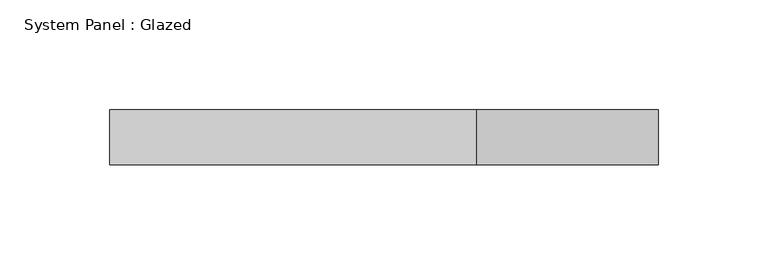
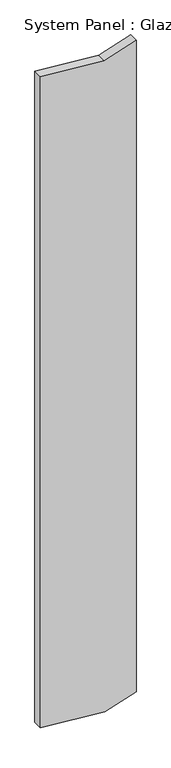
"""IFC4 building model written with IfcOpenShell, lengths in millimetres: plate geometry, System Panel : Glazed."""

import ifcopenshell
import ifcopenshell.guid

model = None  # the IFC model being written
_history = None  # IfcOwnerHistory: only IFC2X3 demands one
_inside = {}  # id of a spatial element -> (the spatial element, [elements in it])
_under = {}  # id of a project, library or spatial element -> (it, [spatial elements below it])
_declared = {}  # id of a project -> (the project, [libraries it declares])
_typed = {}  # id of a type object -> (the type object, [elements of that type])
_made_of = {}  # id of a material, layer set ... -> (it, [elements and type objects made of it])


def new_model(schema):
    """Start an empty IFC model of exactly this schema.

    Asked for "IFC4X3", IfcOpenShell would pick the latest addendum, in which some entities
    have other attributes; the version numbers below select the first issue.
    IFC2X3 requires an IfcOwnerHistory on every rooted entity: one is made here for all.
    """
    global model, _history
    if schema == "IFC4X3":
        model = ifcopenshell.file(schema_version=(4, 3, 0, 0))
    else:
        model = ifcopenshell.file(schema=schema)
    _inside.clear()
    _under.clear()
    _declared.clear()
    _typed.clear()
    _made_of.clear()
    _history = None
    if model.schema == "IFC2X3":
        org = make("IfcOrganization", Name="unknown")
        user = make(
            "IfcPersonAndOrganization",
            ThePerson=make("IfcPerson", FamilyName="unknown"),
            TheOrganization=org,
        )
        app = make(
            "IfcApplication",
            ApplicationDeveloper=org,
            Version="unknown",
            ApplicationFullName="unknown",
            ApplicationIdentifier="unknown",
        )
        _history = make(
            "IfcOwnerHistory",
            OwningUser=user,
            OwningApplication=app,
            ChangeAction="ADDED",
            CreationDate=0,
        )
    return model


def make(cls, **values):
    """One entity of the class cls with the attributes given. An attribute that is None is left unset."""
    return model.create_entity(
        cls, **{name: value for name, value in values.items() if value is not None}
    )


def rooted(cls, **values):
    """An entity with a GlobalId (a new one), such as an element, a storey or a relation."""
    return make(cls, GlobalId=ifcopenshell.guid.new(), OwnerHistory=_history, **values)


def si_unit(unit_type, name, prefix=None):
    """IfcSIUnit, for example si_unit("LENGTHUNIT", "METRE", prefix="MILLI")."""
    return make("IfcSIUnit", UnitType=unit_type, Prefix=prefix, Name=name)


def assignment(units):
    """IfcUnitAssignment: the units of a project."""
    return None if units is None else make("IfcUnitAssignment", Units=units)


def point(xyz):
    """IfcCartesianPoint."""
    return None if xyz is None else make("IfcCartesianPoint", Coordinates=xyz)


def direction(xyz):
    """IfcDirection."""
    return None if xyz is None else make("IfcDirection", DirectionRatios=xyz)


def frame(location, z_axis=None, x_axis=None):
    """IfcAxis2Placement3D, a coordinate frame: its origin and axes. An axis left out is left unset."""
    return make(
        "IfcAxis2Placement3D",
        Location=point(location),
        Axis=direction(z_axis),
        RefDirection=direction(x_axis),
    )


def origin():
    """The frame at (0, 0, 0) with its axes left unset."""
    return frame((0.0, 0.0, 0.0))


def place(relative_to, where):
    """IfcLocalPlacement: puts the frame where relative to a parent placement (None: the world)."""
    return make(
        "IfcLocalPlacement", PlacementRelTo=relative_to, RelativePlacement=where
    )


def context(
    kind, dimensions, precision=None, world=None, true_north=None, identifier=None
):
    """IfcGeometricRepresentationContext, for example the 3D "Model" context."""
    return make(
        "IfcGeometricRepresentationContext",
        ContextIdentifier=identifier,
        ContextType=kind,
        CoordinateSpaceDimension=dimensions,
        Precision=precision,
        WorldCoordinateSystem=world,
        TrueNorth=true_north,
    )


def project(units=None, contexts=None):
    """IfcProject with its units and contexts."""
    return rooted(
        "IfcProject",
        Name="project",
        RepresentationContexts=contexts,
        UnitsInContext=assignment(units),
    )


def spatial(cls, under=None, at=None, **own):
    """A site, building, storey or space (cls), placed at a placement, below another one or the project."""
    s = rooted(cls, ObjectPlacement=at, **own)
    if under is not None:
        _under.setdefault(under.id(), (under, []))[1].append(s)
    return s


def polyline(points):
    """IfcPolyline through the points."""
    return make("IfcPolyline", Points=[point(p) for p in points])


def outline(outer, holes=None, kind="AREA"):
    """IfcArbitraryClosedProfileDef: a profile drawn as a closed curve; with holes, ...WithVoids."""
    if holes is None:
        return make("IfcArbitraryClosedProfileDef", ProfileType=kind, OuterCurve=outer)
    return make(
        "IfcArbitraryProfileDefWithVoids",
        ProfileType=kind,
        OuterCurve=outer,
        InnerCurves=holes,
    )


def extrude(swept, where, along, depth):
    """IfcExtrudedAreaSolid: the profile swept, set in the frame where, extruded along a direction by depth."""
    return make(
        "IfcExtrudedAreaSolid",
        SweptArea=swept,
        Position=where,
        ExtrudedDirection=direction(along),
        Depth=depth,
    )


def shape(context_of_items, identifier, shape_type, items):
    """IfcShapeRepresentation: the items that make up one representation, for example the "Body"."""
    return make(
        "IfcShapeRepresentation",
        ContextOfItems=context_of_items,
        RepresentationIdentifier=identifier,
        RepresentationType=shape_type,
        Items=items,
    )


def source(mapping_origin, context_of_items, identifier, shape_type, items):
    """IfcRepresentationMap: a shape defined once, which mapped items show again and again."""
    return make(
        "IfcRepresentationMap",
        MappingOrigin=mapping_origin,
        MappedRepresentation=shape(context_of_items, identifier, shape_type, items),
    )


def transform(
    local_origin,
    x_axis=None,
    y_axis=None,
    z_axis=None,
    scale=None,
    scale2=None,
    scale3=None,
    uniform=True,
):
    """IfcCartesianTransformationOperator3D, or its non-uniform kind. x_axis, y_axis, z_axis: its Axis1, 2, 3."""
    if uniform:
        return make(
            "IfcCartesianTransformationOperator3D",
            Axis1=direction(x_axis),
            Axis2=direction(y_axis),
            LocalOrigin=point(local_origin),
            Scale=scale,
            Axis3=direction(z_axis),
        )
    return make(
        "IfcCartesianTransformationOperator3DnonUniform",
        Axis1=direction(x_axis),
        Axis2=direction(y_axis),
        LocalOrigin=point(local_origin),
        Scale=scale,
        Axis3=direction(z_axis),
        Scale2=scale2,
        Scale3=scale3,
    )


def mapped(mapping_source, mapping_target):
    """IfcMappedItem: shows the shape of a source again, moved by a transform."""
    return make(
        "IfcMappedItem", MappingSource=mapping_source, MappingTarget=mapping_target
    )


def made_of(thing, what):
    """Note that an element or type object is made of a material, layer set ...; save() writes the relation."""
    if what is not None:
        _made_of.setdefault(what.id(), (what, []))[1].append(thing)
    return thing


def element(
    cls,
    number,
    at=None,
    inside=None,
    cuts=None,
    type_object=None,
    material=None,
    context=None,
    identifier="Body",
    shape_type=None,
    held_by="IfcProductDefinitionShape",
    body=None,
    shapes=None,
    **own,
):
    """One element of the class cls, such as IfcWall. Its Tag is "e" and its number.

    at: its placement. inside: the storey or other place that contains it. cuts: it is an
    opening in that element (IfcRelVoidsElement). A single representation is given by context,
    identifier, shape_type and body (its items); several are given by shapes. held_by: the class
    of the entity that holds the representations. save() writes the other relations.
    """
    e = rooted(cls, Tag="e%d" % number, ObjectPlacement=at, **own)
    if body is not None:
        shapes = [shape(context, identifier, shape_type, body)]
    if shapes is not None:
        e.Representation = make(held_by, Representations=shapes)
    if inside is not None:
        _inside.setdefault(inside.id(), (inside, []))[1].append(e)
    if cuts is not None:
        rooted(
            "IfcRelVoidsElement", RelatingBuildingElement=cuts, RelatedOpeningElement=e
        )
    if type_object is not None:
        _typed.setdefault(type_object.id(), (type_object, []))[1].append(e)
    return made_of(e, material)


def aggregate(whole, parts):
    """IfcRelAggregates: a whole, such as a stair, and the parts it consists of."""
    return rooted("IfcRelAggregates", RelatingObject=whole, RelatedObjects=parts)


def save(model, path):
    """Write the relations noted so far, then the file.

    IfcRelAggregates (storeys below a building ...), IfcRelContainedInSpatialStructure (elements
    in a storey), IfcRelDefinesByType, IfcRelAssociatesMaterial and IfcRelDeclares: one each for
    every whole, place, type object, material and project.
    """
    for whole, parts in _under.values():
        aggregate(whole, parts)
    for where, things in _inside.values():
        rooted(
            "IfcRelContainedInSpatialStructure",
            RelatedElements=things,
            RelatingStructure=where,
        )
    for kind, things in _typed.values():
        rooted("IfcRelDefinesByType", RelatedObjects=things, RelatingType=kind)
    for what, things in _made_of.values():
        rooted("IfcRelAssociatesMaterial", RelatedObjects=things, RelatingMaterial=what)
    for by, libraries in _declared.values():
        rooted("IfcRelDeclares", RelatingContext=by, RelatedDefinitions=libraries)
    model.write(path)


def system_panel_glazed_ad4f34ef(model_context):
    return source(origin(), model_context, "Body", "SweptSolid", [
        extrude(outline(polyline([(14.7138245, -125.0), (0.0, 43.1797838), (27.0254149, 125.0), (1826.3916627, 125.0), (1799.0465952, 42.2120265), (1813.7685539, -125.0), (14.7138245, -125.0)])), frame((0.0, 24.5, 0.0), z_axis=(0.0, 1.0, 0.0), x_axis=(0.0, 0.0, 1.0)), (0.0, 0.0, 1.0), 25.0),
    ])


if __name__ == "__main__":
    model = new_model("IFC4")
    model_context = context("Model", 3, world=origin())
    ifc_project = project(units=[si_unit("LENGTHUNIT", "METRE", prefix="MILLI")], contexts=[model_context])
    site = spatial("IfcSite", under=ifc_project)
    building = spatial("IfcBuilding", under=site)
    placement = place(None, origin())
    system_panel_glazed_shape = system_panel_glazed_ad4f34ef(model_context)
    element("IfcPlate", 1, ObjectType="System Panel : Glazed", at=placement, inside=building, context=model_context, shape_type="MappedRepresentation", body=[
        mapped(system_panel_glazed_shape, transform((0.0, 0.0, 0.0), x_axis=(1.0, 0.0, 0.0), y_axis=(0.0, 1.0, 0.0), z_axis=(0.0, 0.0, 1.0))),
    ])
    save(model, "model.ifc")

# Revit data of these elements
# Element 1 (IfcPlate, "System Panel : Glazed")
#   Materials on its faces: "Glass"
# Materials
#   "Glass": class "Glass", colour RGB 218 227 224, transparency 0.85, Description = "Soda Lime Glass", Cost = 0
